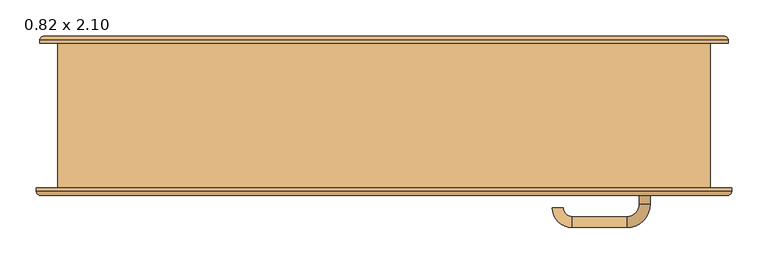
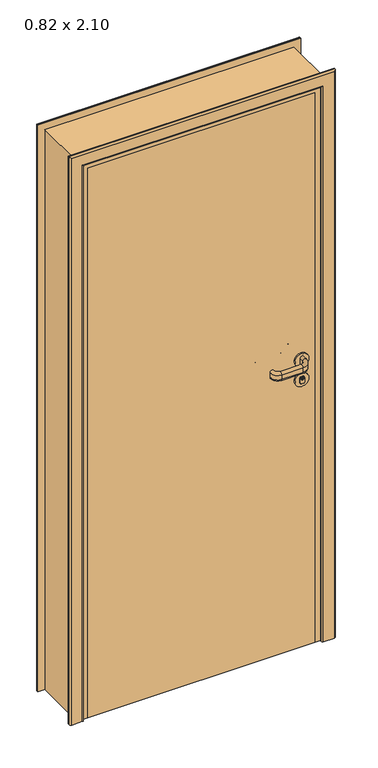
"""IFC4 building model written with IfcOpenShell, lengths in millimetres: door geometry, CC_PORTA ABRIR_1 FOLHA LISA : 0.82 x 2.10."""

from ifc_helpers import new_model, si_unit, point, frame, frame_2d, origin, origin_with_axes, place, context, project, spatial, polyline, circle_curve, ellipse_curve, trimmed, segment, composite_curve, outline, extrude, faceted_brep, source, transform, mapped, element, save
from ifc_brep_helpers import plane_surface, cylinder_surface, revolved_surface, advanced_brep


def door_0_82_x_2_10_bac333eb(model_context):
    return source(origin(), model_context, "Body", "SolidModel", [
        advanced_brep(
        [(352.5, -65.0, 1091.5062746), (367.5, -65.0, 1091.5062746), (367.5, -65.0, 1108.3826844), (352.5, -65.0, 1108.3826844), (367.5, -43.0, 1091.5062746), (367.5, -43.0, 1108.3826844), (352.5, -43.0, 1108.3826844), (352.5, -43.0, 1091.5062746), (335.0, -10.5, 1108.3826844), (335.0, -10.5, 1091.5062746), (260.0, -10.5, 1091.5062746), (260.0, -10.5, 1108.3826844), (335.0, -25.5, 1091.5062746), (335.0, -25.5, 1108.3826844), (260.0, -25.5, 1108.3826844), (260.0, -25.5, 1091.5062746), (247.5, -38.0, 1091.5062746), (247.5, -38.0, 1108.3826844), (232.5, -38.0, 1108.3826844), (232.5, -38.0, 1091.5062746)],
        [
            (0, 1, circle_curve(frame((360.0, -65.0, 1091.5062746), z_axis=(0.0, -1.0, 0.0), x_axis=(0.0, 0.0, 1.0)), 7.5)),
            (1, 2),
            (2, 3, circle_curve(frame((360.0, -65.0, 1108.3826844), z_axis=(0.0, -1.0, 0.0), x_axis=(0.0, 0.0, 1.0)), 7.5)),
            (3, 0),
            (1, 4),
            (4, 5),
            (5, 2),
            (3, 6),
            (6, 7),
            (7, 0),
            (8, 9),
            (9, 10),
            (10, 11),
            (11, 8),
            (12, 13),
            (13, 14),
            (14, 15),
            (15, 12),
            (7, 4, circle_curve(frame((360.0, -43.0, 1091.5062746), z_axis=(0.0, -1.0, 0.0), x_axis=(0.0, 0.0, 1.0)), 7.5)),
            (5, 6, circle_curve(frame((360.0, -43.0, 1108.3826844), z_axis=(0.0, -1.0, 0.0), x_axis=(0.0, 0.0, 1.0)), 7.5)),
            (9, 12, circle_curve(frame((335.0, -18.0, 1091.5062746), z_axis=(-1.0, 0.0, 0.0), x_axis=(0.0, 0.0, 1.0)), 7.5)),
            (15, 10, circle_curve(frame((260.0, -18.0, 1091.5062746), z_axis=(1.0, 0.0, 0.0), x_axis=(0.0, 0.0, 1.0)), 7.5)),
            (13, 8, circle_curve(frame((335.0, -18.0, 1108.3826844), z_axis=(-1.0, 0.0, 0.0), x_axis=(0.0, 0.0, 1.0)), 7.5)),
            (11, 14, circle_curve(frame((260.0, -18.0, 1108.3826844), z_axis=(1.0, 0.0, 0.0), x_axis=(0.0, 0.0, 1.0)), 7.5)),
            (9, 4, circle_curve(frame((335.0, -43.0, 1091.5062746), z_axis=(0.0, 0.0, -1.0), x_axis=(1.0, 0.0, 0.0)), 32.5)),
            (7, 12, circle_curve(frame((335.0, -43.0, 1091.5062746), z_axis=(0.0, 0.0, 1.0), x_axis=(1.0, 0.0, 0.0)), 17.5)),
            (8, 5, circle_curve(frame((335.0, -43.0, 1108.3826844), z_axis=(0.0, 0.0, -1.0), x_axis=(1.0, 0.0, 0.0)), 32.5)),
            (13, 6, circle_curve(frame((335.0, -43.0, 1108.3826844), z_axis=(0.0, 0.0, -1.0), x_axis=(1.0, 0.0, 0.0)), 17.5)),
            (16, 17),
            (17, 18, circle_curve(frame((240.0, -38.0, 1108.3826844), z_axis=(0.0, -1.0, 0.0), x_axis=(0.0, 0.0, 1.0)), 7.5)),
            (18, 19),
            (19, 16, circle_curve(frame((240.0, -38.0, 1091.5062746), z_axis=(0.0, -1.0, 0.0), x_axis=(0.0, 0.0, 1.0)), 7.5)),
            (19, 10, circle_curve(frame((260.0, -38.0, 1091.5062746), z_axis=(0.0, 0.0, -1.0), x_axis=(0.0, 1.0, 0.0)), 27.5)),
            (15, 16, circle_curve(frame((260.0, -38.0, 1091.5062746), z_axis=(0.0, 0.0, 1.0), x_axis=(0.0, 1.0, 0.0)), 12.5)),
            (18, 11, circle_curve(frame((260.0, -38.0, 1108.3826844), z_axis=(0.0, 0.0, -1.0), x_axis=(0.0, 1.0, 0.0)), 27.5)),
            (17, 14, circle_curve(frame((260.0, -38.0, 1108.3826844), z_axis=(0.0, 0.0, -1.0), x_axis=(0.0, 1.0, 0.0)), 12.5)),
        ],
        [
            plane_surface(frame((360.0, -65.0, 1099.9444795), z_axis=(0.0, -1.0, 0.0), x_axis=(0.0, 0.0, 1.0))),
            plane_surface(frame((367.5, -65.0, 1091.5062746), z_axis=(1.0, 0.0, 0.0), x_axis=(0.0, 1.0, 0.0))),
            plane_surface(frame((352.5, -65.0, 1108.3826844), z_axis=(-1.0, 0.0, 0.0), x_axis=(0.0, 1.0, 0.0))),
            plane_surface(frame((335.0, -10.5, 1091.5062746), z_axis=(0.0, 1.0, 0.0), x_axis=(-1.0, 0.0, 0.0))),
            plane_surface(frame((335.0, -25.5, 1108.3826844), z_axis=(0.0, -1.0, 0.0), x_axis=(-1.0, 0.0, 0.0))),
            cylinder_surface(frame((360.0, -65.0, 1091.5062746), z_axis=(0.0, -1.0, 0.0), x_axis=(0.0, 0.0, 1.0)), 7.5),
            cylinder_surface(frame((360.0, -65.0, 1108.3826844), z_axis=(0.0, -1.0, 0.0), x_axis=(0.0, 0.0, 1.0)), 7.5),
            cylinder_surface(frame((335.0, -18.0, 1091.5062746), z_axis=(1.0, 0.0, 0.0), x_axis=(0.0, 0.0, 1.0)), 7.5),
            cylinder_surface(frame((335.0, -18.0, 1108.3826844), z_axis=(1.0, 0.0, 0.0), x_axis=(0.0, 0.0, 1.0)), 7.5),
            revolved_surface(trimmed(ellipse_curve(frame((360.0, -43.0, 1091.5062746), z_axis=(0.0, -1.0, 0.0), x_axis=(0.0, 0.0, 1.0)), 7.5, 7.5), [point((352.5, -43.0, 1091.5062746))], [point((367.5, -43.0, 1091.5062746))], True, "CARTESIAN"), (335.0, -43.0, 1099.9444795), (0.0, 0.0, 1.0)),
            cylinder_surface(frame((335.0, -43.0, 1099.9444795), z_axis=(0.0, 0.0, 1.0), x_axis=(1.0, 0.0, 0.0)), 32.5),
            revolved_surface(trimmed(ellipse_curve(frame((360.0, -43.0, 1108.3826844), z_axis=(0.0, -1.0, 0.0), x_axis=(0.0, 0.0, 1.0)), 7.5, 7.5), [point((367.5, -43.0, 1108.3826844))], [point((352.5, -43.0, 1108.3826844))], True, "CARTESIAN"), (335.0, -43.0, 1099.9444795), (0.0, 0.0, 1.0)),
            revolved_surface(polyline([(352.5, -43.0, 1108.3826844), (352.5, -43.0, 1091.5062746)]), (335.0, -43.0, 1099.9444795), (0.0, 0.0, 1.0)),
            plane_surface(frame((240.0, -38.0, 1099.9444795), z_axis=(0.0, -1.0, 0.0), x_axis=(0.0, 0.0, 1.0))),
            revolved_surface(trimmed(ellipse_curve(frame((260.0, -18.0, 1091.5062746), z_axis=(1.0, 0.0, 0.0), x_axis=(0.0, 0.0, 1.0)), 7.5, 7.5), [point((260.0, -25.5, 1091.5062746))], [point((260.0, -10.5, 1091.5062746))], True, "CARTESIAN"), (260.0, -38.0, 1099.9444795), (0.0, 0.0, 1.0)),
            cylinder_surface(frame((260.0, -38.0, 1099.9444795), z_axis=(0.0, 0.0, 1.0), x_axis=(0.0, 1.0, 0.0)), 27.5),
            revolved_surface(trimmed(ellipse_curve(frame((260.0, -18.0, 1108.3826844), z_axis=(1.0, 0.0, 0.0), x_axis=(0.0, 0.0, 1.0)), 7.5, 7.5), [point((260.0, -10.5, 1108.3826844))], [point((260.0, -25.5, 1108.3826844))], True, "CARTESIAN"), (260.0, -38.0, 1099.9444795), (0.0, 0.0, 1.0)),
            revolved_surface(polyline([(260.0, -25.5, 1108.3826844), (260.0, -25.5, 1091.5062746)]), (260.0, -38.0, 1099.9444795), (0.0, 0.0, 1.0)),
        ],
        [
            (0, [[1, 2, 3, 4]]),
            (1, [[-2, 5, 6, 7]]),
            (2, [[-4, 8, 9, 10]]),
            (3, [[11, 12, 13, 14]]),
            (4, [[15, 16, 17, 18]]),
            (5, [[-1, -10, 19, -5]]),
            (6, [[-3, -7, 20, -8]]),
            (7, [[21, -18, 22, -12]]),
            (8, [[23, -14, 24, -16]]),
            (9, [[25, -19, 26, -21]]),
            (10, [[27, -6, -25, -11]]),
            (11, [[28, -20, -27, -23]]),
            (12, [[-26, -9, -28, -15]]),
            (13, [[29, 30, 31, 32]]),
            (14, [[33, -22, 34, -32]]),
            (15, [[35, -13, -33, -31]]),
            (16, [[36, -24, -35, -30]]),
            (17, [[-34, -17, -36, -29]]),
        ],
    ),
        extrude(outline(polyline([(361.0, -65.0), (359.0, -65.0), (359.0, -55.9), (361.0, -55.9), (361.0, -65.0)])), frame((0.0, 0.0, 1027.9555433), z_axis=(0.0, 0.0, 1.0), x_axis=(1.0, 0.0, 0.0)), (0.0, 0.0, 1.0), 7.8071257),
        extrude(outline(composite_curve([segment(trimmed(circle_curve(frame_2d((1031.5611613, 360.0)), 5.0), [point((1036.5611613, 360.0))], [point((1026.5611613, 360.0))], False, "CARTESIAN"), True, "CONTINUOUS"), segment(trimmed(circle_curve(frame_2d((1031.5611613, 360.0)), 5.0), [point((1026.5611613, 360.0))], [point((1036.5611613, 360.0))], False, "CARTESIAN"), True, "CONTINUOUS")], self_intersect=False), holes=[polyline([(1035.7626689, 361.0), (1027.9555433, 361.0), (1027.9555433, 359.0), (1035.7626689, 359.0), (1035.7626689, 361.0)])]), frame((0.0, -65.0, 0.0), z_axis=(0.0, 1.0, 0.0), x_axis=(0.0, 0.0, 1.0)), (0.0, 0.0, 1.0), 10.0),
        extrude(outline(composite_curve([segment(polyline([(1033.4817325, 352.5), (1016.4817325, 352.5)]), True, "CONTINUOUS"), segment(trimmed(circle_curve(frame_2d((1016.4817325, 356.5)), 4.0), [point((1016.4817325, 352.5))], [point((1012.4817325, 356.5))], False, "CARTESIAN"), True, "CONTINUOUS"), segment(polyline([(1012.4817325, 356.5), (1012.4817325, 363.5)]), True, "CONTINUOUS"), segment(trimmed(circle_curve(frame_2d((1016.4817325, 363.5)), 4.0), [point((1012.4817325, 363.5))], [point((1016.4817325, 367.5))], False, "CARTESIAN"), True, "CONTINUOUS"), segment(polyline([(1016.4817325, 367.5), (1033.4817325, 367.5)]), True, "CONTINUOUS"), segment(trimmed(circle_curve(frame_2d((1033.4817325, 363.5)), 4.0), [point((1033.4817325, 367.5))], [point((1037.4817325, 363.5))], False, "CARTESIAN"), True, "CONTINUOUS"), segment(polyline([(1037.4817325, 363.5), (1037.4817325, 356.5)]), True, "CONTINUOUS"), segment(trimmed(circle_curve(frame_2d((1033.4817325, 356.5)), 4.0), [point((1037.4817325, 356.5))], [point((1033.4817325, 352.5))], False, "CARTESIAN"), True, "CONTINUOUS")], self_intersect=False)), frame((0.0, -65.0, 0.0), z_axis=(0.0, 1.0, 0.0), x_axis=(0.0, 0.0, 1.0)), (0.0, 0.0, 1.0), 9.0),
        extrude(outline(composite_curve([segment(trimmed(circle_curve(frame_2d((1099.9444795, 360.0)), 25.0), [point((1124.9444795, 360.0))], [point((1074.9444795, 360.0))], False, "CARTESIAN"), True, "CONTINUOUS"), segment(trimmed(circle_curve(frame_2d((1099.9444795, 360.0)), 25.0), [point((1074.9444795, 360.0))], [point((1124.9444795, 360.0))], False, "CARTESIAN"), True, "CONTINUOUS")], self_intersect=False)), frame((0.0, -65.0, 0.0), z_axis=(0.0, 1.0, 0.0), x_axis=(0.0, 0.0, 1.0)), (0.0, 0.0, 1.0), 6.0),
        extrude(outline(composite_curve([segment(trimmed(circle_curve(frame_2d((1024.9444795, 360.0)), 25.0), [point((1049.9444795, 360.0))], [point((999.9444795, 360.0))], False, "CARTESIAN"), True, "CONTINUOUS"), segment(trimmed(circle_curve(frame_2d((1024.9444795, 360.0)), 25.0), [point((999.9444795, 360.0))], [point((1049.9444795, 360.0))], False, "CARTESIAN"), True, "CONTINUOUS")], self_intersect=False), holes=[composite_curve([segment(trimmed(circle_curve(frame_2d((1033.4817325, 363.5)), 4.0), [point((1037.4817325, 363.5))], [point((1033.4817325, 367.5))], True, "CARTESIAN"), True, "CONTINUOUS"), segment(polyline([(1033.4817325, 367.5), (1016.4817325, 367.5)]), True, "CONTINUOUS"), segment(trimmed(circle_curve(frame_2d((1016.4817325, 363.5)), 4.0), [point((1016.4817325, 367.5))], [point((1012.4817325, 363.5))], True, "CARTESIAN"), True, "CONTINUOUS"), segment(polyline([(1012.4817325, 363.5), (1012.4817325, 356.5)]), True, "CONTINUOUS"), segment(trimmed(circle_curve(frame_2d((1016.4817325, 356.5)), 4.0), [point((1012.4817325, 356.5))], [point((1016.4817325, 352.5))], True, "CARTESIAN"), True, "CONTINUOUS"), segment(polyline([(1016.4817325, 352.5), (1033.4817325, 352.5)]), True, "CONTINUOUS"), segment(trimmed(circle_curve(frame_2d((1033.4817325, 356.5)), 4.0), [point((1033.4817325, 352.5))], [point((1037.4817325, 356.5))], True, "CARTESIAN"), True, "CONTINUOUS"), segment(polyline([(1037.4817325, 356.5), (1037.4817325, 363.5)]), True, "CONTINUOUS")], self_intersect=False)]), frame((0.0, -65.0, 0.0), z_axis=(0.0, 1.0, 0.0), x_axis=(0.0, 0.0, 1.0)), (0.0, 0.0, 1.0), 6.0),
        extrude(outline(polyline([(361.0, -109.1), (359.0, -109.1), (359.0, -100.0), (361.0, -100.0), (361.0, -109.1)])), frame((0.0, 0.0, 1027.9555433), z_axis=(0.0, 0.0, 1.0), x_axis=(1.0, 0.0, 0.0)), (0.0, 0.0, 1.0), 7.8071257),
        advanced_brep(
        [(360.0, -110.0, 1036.5611613), (360.0, -110.0, 1026.5611613), (361.0, -110.0, 1035.7626689), (361.0, -110.0, 1027.9555433), (359.0, -110.0, 1027.9555433), (359.0, -110.0, 1035.7626689), (360.0, -100.0, 1049.9444795), (360.0, -100.0, 999.9444795), (360.0, -109.0, 1036.5611613), (360.0, -109.0, 1026.5611613), (361.0, -109.0, 1035.7626689), (361.0, -109.0, 1027.9555433), (359.0, -109.0, 1027.9555433), (359.0, -109.0, 1035.7626689), (352.5, -109.0, 1033.4817325), (352.5, -109.0, 1016.4817325), (356.5, -109.0, 1012.4817325), (363.5, -109.0, 1012.4817325), (367.5, -109.0, 1016.4817325), (367.5, -109.0, 1033.4817325), (363.5, -109.0, 1037.4817325), (356.5, -109.0, 1037.4817325), (352.5, -106.0, 1033.4817325), (352.5, -106.0, 1016.4817325), (356.5, -106.0, 1012.4817325), (363.5, -106.0, 1012.4817325), (367.5, -106.0, 1016.4817325), (367.5, -106.0, 1033.4817325), (363.5, -106.0, 1037.4817325), (356.5, -106.0, 1037.4817325), (360.0, -106.0, 1049.9444795), (360.0, -106.0, 999.9444795)],
        [
            (0, 1, circle_curve(frame((360.0, -110.0, 1031.5611613), z_axis=(0.0, -1.0, 0.0), x_axis=(0.0, 0.0, -1.0)), 5.0)),
            (1, 0, circle_curve(frame((360.0, -110.0, 1031.5611613), z_axis=(0.0, -1.0, 0.0), x_axis=(0.0, 0.0, -1.0)), 5.0)),
            (2, 3),
            (3, 4),
            (4, 5),
            (5, 2),
            (6, 7, circle_curve(frame((360.0, -100.0, 1024.9444795), z_axis=(0.0, 1.0, 0.0), x_axis=(0.0, 0.0, -1.0)), 25.0)),
            (7, 6, circle_curve(frame((360.0, -100.0, 1024.9444795), z_axis=(0.0, 1.0, 0.0), x_axis=(0.0, 0.0, -1.0)), 25.0)),
            (0, 8),
            (8, 9, circle_curve(frame((360.0, -109.0, 1031.5611613), z_axis=(0.0, -1.0, 0.0), x_axis=(0.0, 0.0, -1.0)), 5.0)),
            (9, 1),
            (9, 8, circle_curve(frame((360.0, -109.0, 1031.5611613), z_axis=(0.0, -1.0, 0.0), x_axis=(0.0, 0.0, -1.0)), 5.0)),
            (2, 10),
            (10, 11),
            (11, 3),
            (11, 12),
            (12, 4),
            (12, 13),
            (13, 5),
            (13, 10),
            (14, 15),
            (15, 16, circle_curve(frame((356.5, -109.0, 1016.4817325), z_axis=(0.0, -1.0, 0.0), x_axis=(0.0, 0.0, -1.0)), 4.0)),
            (16, 17),
            (17, 18, circle_curve(frame((363.5, -109.0, 1016.4817325), z_axis=(0.0, -1.0, 0.0), x_axis=(0.0, 0.0, -1.0)), 4.0)),
            (18, 19),
            (19, 20, circle_curve(frame((363.5, -109.0, 1033.4817325), z_axis=(0.0, -1.0, 0.0), x_axis=(0.0, 0.0, -1.0)), 4.0)),
            (20, 21),
            (21, 14, circle_curve(frame((356.5, -109.0, 1033.4817325), z_axis=(0.0, -1.0, 0.0), x_axis=(0.0, 0.0, -1.0)), 4.0)),
            (14, 22),
            (22, 23),
            (23, 15),
            (23, 24, circle_curve(frame((356.5, -106.0, 1016.4817325), z_axis=(0.0, -1.0, 0.0), x_axis=(0.0, 0.0, -1.0)), 4.0)),
            (24, 16),
            (24, 25),
            (25, 17),
            (25, 26, circle_curve(frame((363.5, -106.0, 1016.4817325), z_axis=(0.0, -1.0, 0.0), x_axis=(0.0, 0.0, -1.0)), 4.0)),
            (26, 18),
            (26, 27),
            (27, 19),
            (27, 28, circle_curve(frame((363.5, -106.0, 1033.4817325), z_axis=(0.0, -1.0, 0.0), x_axis=(0.0, 0.0, -1.0)), 4.0)),
            (28, 20),
            (28, 29),
            (29, 21),
            (29, 22, circle_curve(frame((356.5, -106.0, 1033.4817325), z_axis=(0.0, -1.0, 0.0), x_axis=(0.0, 0.0, -1.0)), 4.0)),
            (30, 31, circle_curve(frame((360.0, -106.0, 1024.9444795), z_axis=(0.0, -1.0, 0.0), x_axis=(0.0, 0.0, -1.0)), 25.0)),
            (31, 30, circle_curve(frame((360.0, -106.0, 1024.9444795), z_axis=(0.0, -1.0, 0.0), x_axis=(0.0, 0.0, -1.0)), 25.0)),
            (30, 6),
            (7, 31),
        ],
        [
            plane_surface(frame((360.0, -110.0, 1026.5611613), z_axis=(0.0, -1.0, 0.0), x_axis=(1.0, 0.0, 0.0))),
            plane_surface(frame((360.0, -100.0, 1026.5611613), z_axis=(0.0, 1.0, 0.0), x_axis=(-1.0, 0.0, 0.0))),
            cylinder_surface(frame((360.0, -100.0, 1031.5611613), z_axis=(0.0, -1.0, 0.0), x_axis=(0.0, 0.0, -1.0)), 5.0),
            plane_surface(frame((361.0, -110.0, 1035.7626689), z_axis=(-1.0, 0.0, 0.0), x_axis=(0.0, 1.0, 0.0))),
            plane_surface(frame((361.0, -110.0, 1027.9555433), z_axis=(0.0, 0.0, 1.0), x_axis=(0.0, 1.0, 0.0))),
            plane_surface(frame((359.0, -110.0, 1027.9555433), z_axis=(1.0, 0.0, 0.0), x_axis=(0.0, 1.0, 0.0))),
            plane_surface(frame((359.0, -110.0, 1035.7626689), z_axis=(0.0, 0.0, -1.0), x_axis=(0.0, 1.0, 0.0))),
            plane_surface(frame((352.5, -109.0, 1016.4817325), z_axis=(0.0, -1.0, 0.0), x_axis=(0.0, 0.0, -1.0))),
            plane_surface(frame((352.5, -109.0, 1033.4817325), z_axis=(-1.0, 0.0, 0.0), x_axis=(0.0, 1.0, 0.0))),
            cylinder_surface(frame((356.5, -100.0, 1016.4817325), z_axis=(0.0, -1.0, 0.0), x_axis=(0.0, 0.0, -1.0)), 4.0),
            plane_surface(frame((356.5, -109.0, 1012.4817325), z_axis=(0.0, 0.0, -1.0), x_axis=(0.0, 1.0, 0.0))),
            cylinder_surface(frame((363.5, -100.0, 1016.4817325), z_axis=(0.0, -1.0, 0.0), x_axis=(0.0, 0.0, -1.0)), 4.0),
            plane_surface(frame((367.5, -109.0, 1016.4817325), z_axis=(1.0, 0.0, 0.0), x_axis=(0.0, 1.0, 0.0))),
            cylinder_surface(frame((363.5, -100.0, 1033.4817325), z_axis=(0.0, -1.0, 0.0), x_axis=(0.0, 0.0, -1.0)), 4.0),
            plane_surface(frame((363.5, -109.0, 1037.4817325), z_axis=(0.0, 0.0, 1.0), x_axis=(0.0, 1.0, 0.0))),
            cylinder_surface(frame((356.5, -100.0, 1033.4817325), z_axis=(0.0, -1.0, 0.0), x_axis=(0.0, 0.0, -1.0)), 4.0),
            plane_surface(frame((360.0, -106.0, 1074.9444795), z_axis=(0.0, -1.0, 0.0), x_axis=(1.0, 0.0, 0.0))),
            cylinder_surface(frame((360.0, -100.0, 1024.9444795), z_axis=(0.0, -1.0, 0.0), x_axis=(0.0, 0.0, -1.0)), 25.0),
        ],
        [
            (0, [[1, 2], [3, 4, 5, 6]]),
            (1, [[7, 8]]),
            (2, [[-1, 9, 10, 11]]),
            (2, [[-2, -11, 12, -9]]),
            (3, [[-3, 13, 14, 15]]),
            (4, [[-4, -15, 16, 17]]),
            (5, [[-5, -17, 18, 19]]),
            (6, [[-6, -19, 20, -13]]),
            (7, [[-14, -20, -18, -16]]),
            (7, [[21, 22, 23, 24, 25, 26, 27, 28], [-10, -12]]),
            (8, [[-21, 29, 30, 31]]),
            (9, [[-22, -31, 32, 33]]),
            (10, [[-23, -33, 34, 35]]),
            (11, [[-24, -35, 36, 37]]),
            (12, [[-25, -37, 38, 39]]),
            (13, [[-26, -39, 40, 41]]),
            (14, [[-27, -41, 42, 43]]),
            (15, [[-28, -43, 44, -29]]),
            (16, [[45, 46], [-30, -44, -42, -40, -38, -36, -34, -32]]),
            (17, [[-45, 47, -8, 48]]),
            (17, [[-46, -48, -7, -47]]),
        ],
    ),
        advanced_brep(
        [(360.0, -100.0, 1124.9444795), (360.0, -100.0, 1074.9444795), (360.0, -106.0, 1124.9444795), (360.0, -106.0, 1074.9444795)],
        [
            (0, 1, circle_curve(frame((360.0, -100.0, 1099.9444795), z_axis=(0.0, 1.0, 0.0), x_axis=(0.0, 0.0, -1.0)), 25.0)),
            (1, 0, circle_curve(frame((360.0, -100.0, 1099.9444795), z_axis=(0.0, 1.0, 0.0), x_axis=(0.0, 0.0, -1.0)), 25.0)),
            (2, 3, circle_curve(frame((360.0, -106.0, 1099.9444795), z_axis=(0.0, -1.0, 0.0), x_axis=(0.0, 0.0, -1.0)), 25.0)),
            (3, 2, circle_curve(frame((360.0, -106.0, 1099.9444795), z_axis=(0.0, -1.0, 0.0), x_axis=(0.0, 0.0, -1.0)), 25.0)),
            (2, 0),
            (1, 3),
        ],
        [
            plane_surface(frame((360.0, -100.0, 1026.5611613), z_axis=(0.0, 1.0, 0.0), x_axis=(-1.0, 0.0, 0.0))),
            plane_surface(frame((360.0, -106.0, 1074.9444795), z_axis=(0.0, -1.0, 0.0), x_axis=(1.0, 0.0, 0.0))),
            cylinder_surface(frame((360.0, -100.0, 1099.9444795), z_axis=(0.0, -1.0, 0.0), x_axis=(0.0, 0.0, -1.0)), 25.0),
        ],
        [
            (0, [[1, 2]]),
            (1, [[3, 4]]),
            (2, [[-3, 5, -2, 6]]),
            (2, [[-4, -6, -1, -5]]),
        ],
    ),
        advanced_brep(
        [(352.5, -100.0, 1108.4382049), (367.5, -100.0, 1108.4382049), (367.5, -100.0, 1091.5617951), (352.5, -100.0, 1091.5617951), (367.5, -122.0, 1108.4382049), (367.5, -122.0, 1091.5617951), (352.5, -122.0, 1091.5617951), (352.5, -122.0, 1108.4382049), (335.0, -154.5, 1091.5617951), (335.0, -154.5, 1108.4382049), (260.0, -154.5, 1108.4382049), (260.0, -154.5, 1091.5617951), (335.0, -139.5, 1108.4382049), (335.0, -139.5, 1091.5617951), (260.0, -139.5, 1091.5617951), (260.0, -139.5, 1108.4382049), (247.5, -127.0, 1108.4382049), (247.5, -127.0, 1091.5617951), (232.5, -127.0, 1091.5617951), (232.5, -127.0, 1108.4382049)],
        [
            (0, 1, circle_curve(frame((360.0, -100.0, 1108.4382049), z_axis=(0.0, 1.0, 0.0), x_axis=(-1.0, 0.0, 0.0)), 7.5)),
            (1, 2),
            (2, 3, circle_curve(frame((360.0, -100.0, 1091.5617951), z_axis=(0.0, 1.0, 0.0), x_axis=(-1.0, 0.0, 0.0)), 7.5)),
            (3, 0),
            (1, 4),
            (4, 5),
            (5, 2),
            (3, 6),
            (6, 7),
            (7, 0),
            (8, 9),
            (9, 10),
            (10, 11),
            (11, 8),
            (12, 13),
            (13, 14),
            (14, 15),
            (15, 12),
            (7, 4, circle_curve(frame((360.0, -122.0, 1108.4382049), z_axis=(0.0, 1.0, 0.0), x_axis=(-1.0, 0.0, 0.0)), 7.5)),
            (5, 6, circle_curve(frame((360.0, -122.0, 1091.5617951), z_axis=(0.0, 1.0, 0.0), x_axis=(-1.0, 0.0, 0.0)), 7.5)),
            (9, 12, circle_curve(frame((335.0, -147.0, 1108.4382049), z_axis=(-1.0, 0.0, 0.0), x_axis=(0.0, 1.0, 0.0)), 7.5)),
            (15, 10, circle_curve(frame((260.0, -147.0, 1108.4382049), z_axis=(1.0, 0.0, 0.0), x_axis=(0.0, 1.0, 0.0)), 7.5)),
            (13, 8, circle_curve(frame((335.0, -147.0, 1091.5617951), z_axis=(-1.0, 0.0, 0.0), x_axis=(0.0, 1.0, 0.0)), 7.5)),
            (11, 14, circle_curve(frame((260.0, -147.0, 1091.5617951), z_axis=(1.0, 0.0, 0.0), x_axis=(0.0, 1.0, 0.0)), 7.5)),
            (9, 4, circle_curve(frame((335.0, -122.0, 1108.4382049), z_axis=(0.0, 0.0, 1.0), x_axis=(1.0, 0.0, 0.0)), 32.5)),
            (7, 12, circle_curve(frame((335.0, -122.0, 1108.4382049), z_axis=(0.0, 0.0, -1.0), x_axis=(1.0, 0.0, 0.0)), 17.5)),
            (8, 5, circle_curve(frame((335.0, -122.0, 1091.5617951), z_axis=(0.0, 0.0, 1.0), x_axis=(1.0, 0.0, 0.0)), 32.5)),
            (13, 6, circle_curve(frame((335.0, -122.0, 1091.5617951), z_axis=(0.0, 0.0, 1.0), x_axis=(1.0, 0.0, 0.0)), 17.5)),
            (16, 17),
            (17, 18, circle_curve(frame((240.0, -127.0, 1091.5617951), z_axis=(0.0, 1.0, 0.0), x_axis=(1.0, 0.0, 0.0)), 7.5)),
            (18, 19),
            (19, 16, circle_curve(frame((240.0, -127.0, 1108.4382049), z_axis=(0.0, 1.0, 0.0), x_axis=(1.0, 0.0, 0.0)), 7.5)),
            (19, 10, circle_curve(frame((260.0, -127.0, 1108.4382049), z_axis=(0.0, 0.0, 1.0), x_axis=(0.0, -1.0, 0.0)), 27.5)),
            (15, 16, circle_curve(frame((260.0, -127.0, 1108.4382049), z_axis=(0.0, 0.0, -1.0), x_axis=(0.0, -1.0, 0.0)), 12.5)),
            (18, 11, circle_curve(frame((260.0, -127.0, 1091.5617951), z_axis=(0.0, 0.0, 1.0), x_axis=(0.0, -1.0, 0.0)), 27.5)),
            (17, 14, circle_curve(frame((260.0, -127.0, 1091.5617951), z_axis=(0.0, 0.0, 1.0), x_axis=(0.0, -1.0, 0.0)), 12.5)),
        ],
        [
            plane_surface(frame((360.0, -100.0, 1100.0), z_axis=(0.0, 1.0, 0.0), x_axis=(0.0, 0.0, -1.0))),
            plane_surface(frame((367.5, -100.0, 1108.4382049), z_axis=(1.0, 0.0, 0.0), x_axis=(0.0, -1.0, 0.0))),
            plane_surface(frame((352.5, -100.0, 1091.5617951), z_axis=(-1.0, 0.0, 0.0), x_axis=(0.0, -1.0, 0.0))),
            plane_surface(frame((335.0, -154.5, 1108.4382049), z_axis=(0.0, -1.0, 0.0), x_axis=(-1.0, 0.0, 0.0))),
            plane_surface(frame((335.0, -139.5, 1091.5617951), z_axis=(0.0, 1.0, 0.0), x_axis=(-1.0, 0.0, 0.0))),
            cylinder_surface(frame((360.0, -100.0, 1108.4382049), z_axis=(0.0, 1.0, 0.0), x_axis=(-1.0, 0.0, 0.0)), 7.5),
            cylinder_surface(frame((360.0, -100.0, 1091.5617951), z_axis=(0.0, 1.0, 0.0), x_axis=(-1.0, 0.0, 0.0)), 7.5),
            cylinder_surface(frame((335.0, -147.0, 1108.4382049), z_axis=(1.0, 0.0, 0.0), x_axis=(0.0, 1.0, 0.0)), 7.5),
            cylinder_surface(frame((335.0, -147.0, 1091.5617951), z_axis=(1.0, 0.0, 0.0), x_axis=(0.0, 1.0, 0.0)), 7.5),
            revolved_surface(trimmed(ellipse_curve(frame((360.0, -122.0, 1108.4382049), z_axis=(0.0, 1.0, 0.0), x_axis=(-1.0, 0.0, 0.0)), 7.5, 7.5), [point((352.5, -122.0, 1108.4382049))], [point((367.5, -122.0, 1108.4382049))], True, "CARTESIAN"), (335.0, -122.0, 1100.0), (0.0, 0.0, -1.0)),
            cylinder_surface(frame((335.0, -122.0, 1100.0), z_axis=(0.0, 0.0, -1.0), x_axis=(1.0, 0.0, 0.0)), 32.5),
            revolved_surface(trimmed(ellipse_curve(frame((360.0, -122.0, 1091.5617951), z_axis=(0.0, 1.0, 0.0), x_axis=(-1.0, 0.0, 0.0)), 7.5, 7.5), [point((367.5, -122.0, 1091.5617951))], [point((352.5, -122.0, 1091.5617951))], True, "CARTESIAN"), (335.0, -122.0, 1100.0), (0.0, 0.0, -1.0)),
            revolved_surface(polyline([(352.5, -122.0, 1091.5617951), (352.5, -122.0, 1108.4382049)]), (335.0, -122.0, 1100.0), (0.0, 0.0, -1.0)),
            plane_surface(frame((240.0, -127.0, 1100.0), z_axis=(0.0, 1.0, 0.0), x_axis=(0.0, 0.0, -1.0))),
            revolved_surface(trimmed(ellipse_curve(frame((260.0, -147.0, 1108.4382049), z_axis=(1.0, 0.0, 0.0), x_axis=(0.0, 1.0, 0.0)), 7.5, 7.5), [point((260.0, -139.5, 1108.4382049))], [point((260.0, -154.5, 1108.4382049))], True, "CARTESIAN"), (260.0, -127.0, 1100.0), (0.0, 0.0, -1.0)),
            cylinder_surface(frame((260.0, -127.0, 1100.0), z_axis=(0.0, 0.0, -1.0), x_axis=(0.0, -1.0, 0.0)), 27.5),
            revolved_surface(trimmed(ellipse_curve(frame((260.0, -147.0, 1091.5617951), z_axis=(1.0, 0.0, 0.0), x_axis=(0.0, 1.0, 0.0)), 7.5, 7.5), [point((260.0, -154.5, 1091.5617951))], [point((260.0, -139.5, 1091.5617951))], True, "CARTESIAN"), (260.0, -127.0, 1100.0), (0.0, 0.0, -1.0)),
            revolved_surface(polyline([(260.0, -139.5, 1091.5617951), (260.0, -139.5, 1108.4382049)]), (260.0, -127.0, 1100.0), (0.0, 0.0, -1.0)),
        ],
        [
            (0, [[1, 2, 3, 4]]),
            (1, [[-2, 5, 6, 7]]),
            (2, [[-4, 8, 9, 10]]),
            (3, [[11, 12, 13, 14]]),
            (4, [[15, 16, 17, 18]]),
            (5, [[-1, -10, 19, -5]]),
            (6, [[-3, -7, 20, -8]]),
            (7, [[21, -18, 22, -12]]),
            (8, [[23, -14, 24, -16]]),
            (9, [[25, -19, 26, -21]]),
            (10, [[27, -6, -25, -11]]),
            (11, [[28, -20, -27, -23]]),
            (12, [[-26, -9, -28, -15]]),
            (13, [[29, 30, 31, 32]]),
            (14, [[33, -22, 34, -32]]),
            (15, [[35, -13, -33, -31]]),
            (16, [[36, -24, -35, -30]]),
            (17, [[-34, -17, -36, -29]]),
        ],
    ),
        extrude(outline(polyline([(410.0, -100.0), (-410.0, -100.0), (-410.0, -65.0), (410.0, -65.0), (410.0, -100.0)])), origin_with_axes(), (0.0, 0.0, 1.0), 2100.0),
        advanced_brep(
        [(-430.5, 110.0, 0.0), (-425.0, 104.5, 0.0), (-425.0, 100.0, 0.0), (-475.0, 100.0, 0.0), (-475.0, 104.500573, 0.0), (-469.500573, 110.0, 0.0), (-430.5, 110.0, 2120.5), (-425.0, 104.5, 2115.0), (-425.0, 100.0, 2115.0), (425.0, 100.0, 2115.0), (425.0, 100.0, 0.0), (475.0, 100.0, 0.0), (475.0, 100.0, 2165.0), (-475.0, 100.0, 2165.0), (-475.0, 104.500573, 2165.0), (-469.500573, 110.0, 2159.500573), (469.500573, 110.0, 2159.500573), (469.500573, 110.0, 0.0), (430.5, 110.0, 0.0), (430.5, 110.0, 2120.5), (425.0, 104.5, 2115.0), (425.0, 104.5, 0.0), (475.0, 104.500573, 0.0), (475.0, 104.500573, 2165.0)],
        [
            (0, 1, circle_curve(frame((-430.5, 104.5, 0.0), z_axis=(0.0, 0.0, -1.0), x_axis=(0.0, 1.0, 0.0)), 5.5)),
            (1, 2),
            (2, 3),
            (3, 4),
            (4, 5, circle_curve(frame((-469.500573, 104.500573, 0.0), z_axis=(0.0, 0.0, -1.0), x_axis=(0.0, 1.0, 0.0)), 5.499427)),
            (5, 0),
            (0, 6),
            (6, 7, ellipse_curve(frame((-430.5, 104.5, 2120.5), z_axis=(-0.7071067811865475, 0.0, -0.7071067811865475), x_axis=(0.7071067811865474, 0.0, -0.7071067811865476)), 7.7781746, 5.5)),
            (7, 1),
            (7, 8),
            (8, 2),
            (8, 9),
            (9, 10),
            (10, 11),
            (11, 12),
            (12, 13),
            (13, 3),
            (13, 14),
            (14, 4),
            (14, 15, ellipse_curve(frame((-469.500573, 104.500573, 2159.500573), z_axis=(-0.7071067811865475, 0.0, -0.7071067811865475), x_axis=(0.7071067811865474, 0.0, -0.7071067811865476)), 7.7773642, 5.499427)),
            (15, 5),
            (15, 16),
            (16, 17),
            (17, 18),
            (18, 19),
            (19, 6),
            (9, 20),
            (20, 21),
            (21, 10),
            (17, 22, circle_curve(frame((469.500573, 104.500573, 0.0), z_axis=(0.0, 0.0, -1.0), x_axis=(0.0, 1.0, 0.0)), 5.499427)),
            (22, 11),
            (21, 18, circle_curve(frame((430.5, 104.5, 0.0), z_axis=(0.0, 0.0, -1.0), x_axis=(0.0, 1.0, 0.0)), 5.5)),
            (23, 12),
            (22, 23),
            (16, 23, ellipse_curve(frame((469.500573, 104.500573, 2159.500573), z_axis=(0.7071067811865475, 0.0, -0.7071067811865475), x_axis=(0.7071067811865474, 0.0, 0.7071067811865476)), 7.7773642, 5.499427)),
            (20, 19, ellipse_curve(frame((430.5, 104.5, 2120.5), z_axis=(0.7071067811865475, 0.0, -0.7071067811865475), x_axis=(0.7071067811865474, 0.0, 0.7071067811865476)), 7.7781746, 5.5)),
            (20, 7),
            (23, 14),
        ],
        [
            plane_surface(frame((-450.0, 100.0, 0.0), z_axis=(0.0, 0.0, -1.0), x_axis=(-1.0, 0.0, 0.0))),
            cylinder_surface(frame((-430.5, 104.5, 0.0), z_axis=(0.0, 0.0, -1.0), x_axis=(0.0, 1.0, 0.0)), 5.5),
            plane_surface(frame((-425.0, 104.5, 0.0), z_axis=(1.0, 0.0, 0.0), x_axis=(0.0, 0.0, 1.0))),
            plane_surface(frame((-425.0, 100.0, 0.0), z_axis=(0.0, -1.0, 0.0), x_axis=(0.0, 0.0, 1.0))),
            plane_surface(frame((-475.0, 100.0, 0.0), z_axis=(-1.0, 0.0, 0.0), x_axis=(0.0, 0.0, 1.0))),
            cylinder_surface(frame((-469.500573, 104.500573, 0.0), z_axis=(0.0, 0.0, -1.0), x_axis=(0.0, 1.0, 0.0)), 5.499427),
            plane_surface(frame((-469.500573, 110.0, 0.0), z_axis=(0.0, 1.0, 0.0), x_axis=(0.0, 0.0, 1.0))),
            plane_surface(frame((425.0, 104.5, 2115.0), z_axis=(-1.0, 0.0, 0.0), x_axis=(0.0, 0.0, -1.0))),
            plane_surface(frame((450.0, 100.0, 0.0), z_axis=(0.0, 0.0, -1.0), x_axis=(1.0, 0.0, 0.0))),
            plane_surface(frame((475.0, 100.0, 2165.0), z_axis=(1.0, 0.0, 0.0), x_axis=(0.0, 0.0, -1.0))),
            cylinder_surface(frame((469.500573, 104.500573, 2140.0), z_axis=(0.0, 0.0, 1.0), x_axis=(0.0, 1.0, 0.0)), 5.499427),
            cylinder_surface(frame((430.5, 104.5, 2140.0), z_axis=(0.0, 0.0, 1.0), x_axis=(0.0, 1.0, 0.0)), 5.5),
            cylinder_surface(frame((-450.0, 104.5, 2120.5), z_axis=(-1.0, 0.0, 0.0), x_axis=(0.0, 1.0, 0.0)), 5.5),
            plane_surface(frame((-425.0, 104.5, 2115.0), z_axis=(0.0, 0.0, -1.0), x_axis=(1.0, 0.0, 0.0))),
            plane_surface(frame((-475.0, 100.0, 2165.0), z_axis=(0.0, 0.0, 1.0), x_axis=(1.0, 0.0, 0.0))),
            cylinder_surface(frame((-450.0, 104.500573, 2159.500573), z_axis=(-1.0, 0.0, 0.0), x_axis=(0.0, 1.0, 0.0)), 5.499427),
        ],
        [
            (0, [[1, 2, 3, 4, 5, 6]]),
            (1, [[-1, 7, 8, 9]]),
            (2, [[-2, -9, 10, 11]]),
            (3, [[-3, -11, 12, 13, 14, 15, 16, 17]]),
            (4, [[-4, -17, 18, 19]]),
            (5, [[-5, -19, 20, 21]]),
            (6, [[-6, -21, 22, 23, 24, 25, 26, -7]]),
            (7, [[27, 28, 29, -13]]),
            (8, [[-24, 30, 31, -14, -29, 32]]),
            (9, [[33, -15, -31, 34]]),
            (10, [[35, -34, -30, -23]]),
            (11, [[36, -25, -32, -28]]),
            (12, [[-8, -26, -36, 37]]),
            (13, [[-10, -37, -27, -12]]),
            (14, [[-18, -16, -33, 38]]),
            (15, [[-20, -38, -35, -22]]),
        ],
    ),
        advanced_brep(
        [(-430.0, -100.0, 0.0), (-430.0, -104.5, 0.0), (-435.5, -110.0, 0.0), (-474.5, -110.0, 0.0), (-480.0, -104.5, 0.0), (-480.0, -100.0, 0.0), (-430.0, -100.0, 2120.0), (-430.0, -104.5, 2120.0), (-435.5, -110.0, 2125.5), (435.5, -110.0, 2125.5), (435.5, -110.0, 0.0), (474.5, -110.0, 0.0), (474.5, -110.0, 2164.5), (-474.5, -110.0, 2164.5), (-480.0, -104.5, 2170.0), (-480.0, -100.0, 2170.0), (480.0, -100.0, 2170.0), (480.0, -100.0, 0.0), (430.0, -100.0, 0.0), (430.0, -100.0, 2120.0), (430.0, -104.5, 2120.0), (430.0, -104.5, 0.0), (480.0, -104.5, 0.0), (480.0, -104.5, 2170.0)],
        [
            (0, 1),
            (1, 2, circle_curve(frame((-435.5, -104.5, 0.0), z_axis=(0.0, 0.0, -1.0), x_axis=(0.0, 1.0, 0.0)), 5.5)),
            (2, 3),
            (3, 4, circle_curve(frame((-474.5, -104.5, 0.0), z_axis=(0.0, 0.0, -1.0), x_axis=(0.0, 1.0, 0.0)), 5.5)),
            (4, 5),
            (5, 0),
            (0, 6),
            (6, 7),
            (7, 1),
            (7, 8, ellipse_curve(frame((-435.5, -104.5, 2125.5), z_axis=(-0.7071067811865475, 0.0, -0.7071067811865475), x_axis=(0.7071067811865474, 0.0, -0.7071067811865476)), 7.7781746, 5.5)),
            (8, 2),
            (8, 9),
            (9, 10),
            (10, 11),
            (11, 12),
            (12, 13),
            (13, 3),
            (13, 14, ellipse_curve(frame((-474.5, -104.5, 2164.5), z_axis=(-0.7071067811865475, 0.0, -0.7071067811865475), x_axis=(0.7071067811865474, 0.0, -0.7071067811865476)), 7.7781746, 5.5)),
            (14, 4),
            (14, 15),
            (15, 5),
            (15, 16),
            (16, 17),
            (17, 18),
            (18, 19),
            (19, 6),
            (9, 20, ellipse_curve(frame((435.5, -104.5, 2125.5), z_axis=(0.7071067811865475, 0.0, -0.7071067811865475), x_axis=(0.7071067811865474, 0.0, 0.7071067811865476)), 7.7781746, 5.5)),
            (20, 21),
            (21, 10, circle_curve(frame((435.5, -104.5, 0.0), z_axis=(0.0, 0.0, 1.0), x_axis=(0.0, 1.0, 0.0)), 5.5)),
            (17, 22),
            (22, 11, circle_curve(frame((474.5, -104.5, 0.0), z_axis=(0.0, 0.0, -1.0), x_axis=(0.0, 1.0, 0.0)), 5.5)),
            (21, 18),
            (23, 12, ellipse_curve(frame((474.5, -104.5, 2164.5), z_axis=(0.7071067811865475, 0.0, -0.7071067811865475), x_axis=(0.7071067811865474, 0.0, 0.7071067811865476)), 7.7781746, 5.5)),
            (22, 23),
            (16, 23),
            (20, 19),
            (20, 7),
            (23, 14),
        ],
        [
            plane_surface(frame((-450.0, -100.0, 0.0), z_axis=(0.0, 0.0, -1.0), x_axis=(-1.0, 0.0, 0.0))),
            plane_surface(frame((-430.0, -100.0, 0.0), z_axis=(1.0, 0.0, 0.0), x_axis=(0.0, 0.0, 1.0))),
            cylinder_surface(frame((-435.5, -104.5, 0.0), z_axis=(0.0, 0.0, -1.0), x_axis=(0.0, 1.0, 0.0)), 5.5),
            plane_surface(frame((-435.5, -110.0, 0.0), z_axis=(0.0, -1.0, 0.0), x_axis=(0.0, 0.0, 1.0))),
            cylinder_surface(frame((-474.5, -104.5, 0.0), z_axis=(0.0, 0.0, -1.0), x_axis=(0.0, 1.0, 0.0)), 5.5),
            plane_surface(frame((-480.0, -104.5, 0.0), z_axis=(-1.0, 0.0, 0.0), x_axis=(0.0, 0.0, 1.0))),
            plane_surface(frame((-480.0, -100.0, 0.0), z_axis=(0.0, 1.0, 0.0), x_axis=(0.0, 0.0, 1.0))),
            cylinder_surface(frame((435.5, -104.5, 2140.0), z_axis=(0.0, 0.0, 1.0), x_axis=(0.0, 1.0, 0.0)), 5.5),
            plane_surface(frame((450.0, -100.0, 0.0), z_axis=(0.0, 0.0, -1.0), x_axis=(1.0, 0.0, 0.0))),
            cylinder_surface(frame((474.5, -104.5, 2140.0), z_axis=(0.0, 0.0, 1.0), x_axis=(0.0, 1.0, 0.0)), 5.5),
            plane_surface(frame((480.0, -104.5, 2170.0), z_axis=(1.0, 0.0, 0.0), x_axis=(0.0, 0.0, -1.0))),
            plane_surface(frame((430.0, -100.0, 2120.0), z_axis=(-1.0, 0.0, 0.0), x_axis=(0.0, 0.0, -1.0))),
            plane_surface(frame((-430.0, -100.0, 2120.0), z_axis=(0.0, 0.0, -1.0), x_axis=(1.0, 0.0, 0.0))),
            cylinder_surface(frame((-450.0, -104.5, 2125.5), z_axis=(-1.0, 0.0, 0.0), x_axis=(0.0, 1.0, 0.0)), 5.5),
            cylinder_surface(frame((-450.0, -104.5, 2164.5), z_axis=(-1.0, 0.0, 0.0), x_axis=(0.0, 1.0, 0.0)), 5.5),
            plane_surface(frame((-480.0, -104.5, 2170.0), z_axis=(0.0, 0.0, 1.0), x_axis=(1.0, 0.0, 0.0))),
        ],
        [
            (0, [[1, 2, 3, 4, 5, 6]]),
            (1, [[-1, 7, 8, 9]]),
            (2, [[-2, -9, 10, 11]]),
            (3, [[-3, -11, 12, 13, 14, 15, 16, 17]]),
            (4, [[-4, -17, 18, 19]]),
            (5, [[-5, -19, 20, 21]]),
            (6, [[-6, -21, 22, 23, 24, 25, 26, -7]]),
            (7, [[27, 28, 29, -13]]),
            (8, [[-24, 30, 31, -14, -29, 32]]),
            (9, [[33, -15, -31, 34]]),
            (10, [[35, -34, -30, -23]]),
            (11, [[36, -25, -32, -28]]),
            (12, [[-8, -26, -36, 37]]),
            (13, [[-10, -37, -27, -12]]),
            (14, [[-18, -16, -33, 38]]),
            (15, [[-20, -38, -35, -22]]),
        ],
    ),
        faceted_brep([(-410.0, -65.0, 0.0), (-410.0, -100.0, 0.0), (-450.0, -100.0, 0.0), (-450.0, 100.0, 0.0), (-400.0, 100.0, 0.0), (-400.0, -65.0, 0.0), (-410.0, -65.0, 2100.0), (-410.0, -100.0, 2100.0), (410.0, -100.0, 2100.0), (410.0, -100.0, 0.0), (450.0, -100.0, 0.0), (450.0, -100.0, 2140.0), (-450.0, -100.0, 2140.0), (-450.0, 100.0, 2140.0), (450.0, 100.0, 2140.0), (450.0, 100.0, 0.0), (400.0, 100.0, 0.0), (400.0, 100.0, 2090.0), (-400.0, 100.0, 2090.0), (-400.0, -65.0, 2090.0), (400.0, -65.0, 2090.0), (400.0, -65.0, 0.0), (410.0, -65.0, 0.0), (410.0, -65.0, 2100.0)], [[[0, 1, 2, 3, 4, 5]], [[1, 0, 6, 7]], [[2, 1, 7, 8, 9, 10, 11, 12]], [[3, 2, 12, 13]], [[4, 3, 13, 14, 15, 16, 17, 18]], [[5, 4, 18, 19]], [[0, 5, 19, 20, 21, 22, 23, 6]], [[8, 23, 22, 9]], [[22, 21, 16, 15, 10, 9]], [[14, 11, 10, 15]], [[20, 17, 16, 21]], [[7, 6, 23, 8]], [[13, 12, 11, 14]], [[19, 18, 17, 20]]]),
    ])


if __name__ == "__main__":
    model = new_model("IFC4")
    model_context = context("Model", 3, world=origin())
    ifc_project = project(units=[si_unit("LENGTHUNIT", "METRE", prefix="MILLI")], contexts=[model_context])
    site = spatial("IfcSite", under=ifc_project)
    building = spatial("IfcBuilding", under=site)
    placement = place(None, origin())
    door_0_82_x_2_10_shape = door_0_82_x_2_10_bac333eb(model_context)
    element("IfcDoor", 1, ObjectType="CC_PORTA ABRIR_1 FOLHA LISA : 0.82 x 2.10", at=placement, inside=building, context=model_context, shape_type="MappedRepresentation", body=[
        mapped(door_0_82_x_2_10_shape, transform((0.0, 0.0, 0.0), x_axis=(1.0, 0.0, 0.0), y_axis=(0.0, 1.0, 0.0), z_axis=(0.0, 0.0, 1.0))),
    ])
    save(model, "model.ifc")

# Revit data of these elements
# Type "CC_PORTA ABRIR_1 FOLHA LISA : 0.82 x 2.10"
#   Type Mark = "P6"
#   Site = "www.construir.arq.br"
#   Empresa = "Cursos Construir"
#   Description = "PORTA ABRIR 1 FOLHA LISA"
#   Criado Por = "Roberto Netto"
#   Analytic Construction = "<Nenhum>"
#   Atualizado por = "Rudemberg Eloi"
#   Rough Width = 0.90 m
#   Interna [instance default] = 0.00 m
#   Largura Guarnição Interna [instance default] = 0.05 m
#   Largura Guarnição Externa [instance default] = 0.05 m
#   Largura Folha [instance default] = 0.82 m
#   Externa [instance default] = 0.00 m
#   Extensão Lateral Esquerda [instance default] = 0.03 m
#   Extensão Lateral Direita [instance default] = 0.03 m
#   Extensão Frontal [instance default] = 0.03 m
#   Espessura Soleira [instance default] = 0.02 m
#   Espessura Guarnição Interna [instance default] = 0.01 m
#   Espessura Guarnição Externa [instance default] = 0.01 m
#   Espessura Folha [instance default] = 0.035 m
#   Espessura Batente [instance default] = 0.05 m
#   Eixo Rotação Folha [instance default] = 0.04 m
#   Deslocamento Maçaneta [instance default] = 0.05 m
#   Deslocamento Fechadura [instance default] = 0.05 m
#   Desloc (Interno) [instance default] = 0.02 m
#   Desloc (Externo) [instance default] = 0.025 m
#   Rough Height = 2.14 m
#   Altura Maçaneta [instance default] = 1.10 m
#   Altura Folha [instance default] = 2.10 m
#   Altura Fechadura [instance default] = 1.00 m
#   Height = 2.14 m
#   Width = 0.90 m
#   ----SOLEIRA---- [instance default] = 0.00 m
#   ----MAÇANETA/FECHADURA---- [instance default] = 0.00 m
#   ----GUARNIÇÃO---- [instance default] = 0.00 m
#   ----FOLHA---- [instance default] = 0.00 m
#   ----EXTENSÃO---- [instance default] = 0.00 m
#   ----BATENTE---- [instance default] = 0.00 m
#   Soleira Sem Extensão [instance default] = yes
#   Soleira Com Extensão [instance default] = no
#   Soleira [instance default] = yes
#   Maçaneta / Puxador [instance default] = yes
#   Guarnição Interna [instance default] = yes
#   Guarnição Externa [instance default] = yes
#   Fechadura Separada [instance default] = no
#   Bit [instance default] = no
#   Porcent. Exibição Batente Interno [instance default] = 50
#   Porcent. Exibição Batente Externo [instance default] = 50
#   Material Bit/Soleira = .GRANITO BRANCO ITAÚNAS
#   Material Espelho/Fixação = .AÇO INOXIDÁVEL ESCOVADO
#   Material Maçaneta/Puxador = .AÇO INOXIDÁVEL ESCOVADO
#   Material Guarnição Interna = .MADEIRA COM PINTURA ESMALTE BRANCO ACETINADO
#   Material Guarnição Externa = .MADEIRA COM PINTURA ESMALTE BRANCO ACETINADO
#   Material Folha = .MADEIRA COM PINTURA ESMALTE BRANCO ACETINADO
#   Material Fechadura = .AÇO INOXIDÁVEL ESCOVADO
#   Material Batente = .MADEIRA COM PINTURA ESMALTE BRANCO ACETINADO
#   Família Maçaneta [instance default] = element 1947931
#   Function = (empty or 0)
#   Wall Closure = (empty or 0)
# Element 1 (IfcDoor, "CC_PORTA ABRIR_1 FOLHA LISA : 0.82 x 2.10")
#   Materials on its faces: ".AÇO INOXIDÁVEL ESCOVADO", ".MADEIRA COM PINTURA ESMALTE BRANCO ACETINADO"
# Materials
#   ".GRANITO BRANCO ITAÚNAS": class ".CC_PEDRA REVEST.", colour RGB 202 195 174, transparency 0, Description = "Granito branco Itaúnas", Uso = "Pedra", Cost = 0
#   ".AÇO INOXIDÁVEL ESCOVADO": class "Metal", colour RGB 189 187 185, transparency 0, Description = "Stainless Steel 18/8, brushed finish", Cost = 0
#   ".MADEIRA COM PINTURA ESMALTE BRANCO ACETINADO": class ".CC_MADEIRAS", colour RGB 240 240 240, transparency 0, Description = "Madeira com pintura esmalte branco acetinado.", Cost = 0
